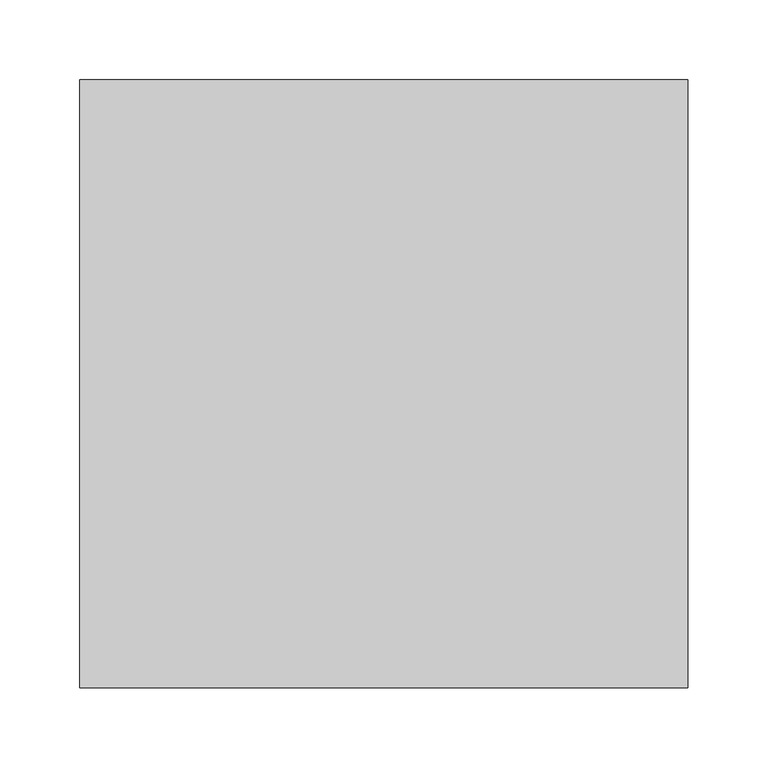
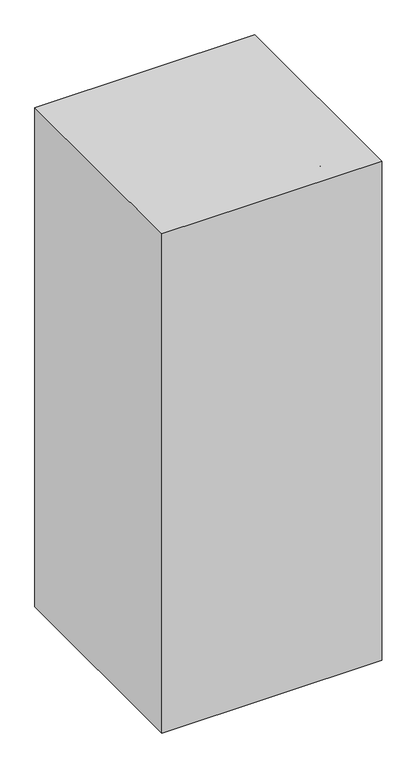
"""IFC4 building model written with IfcOpenShell, lengths in millimetres: proxy geometry, P2000 - Eyewash, Wall Mounted, Hands-Free : P2000 - Eyewash, Wall Mounted, Hands-Free."""

import ifcopenshell
import ifcopenshell.guid

model = None  # the IFC model being written
_history = None  # IfcOwnerHistory: only IFC2X3 demands one
_inside = {}  # id of a spatial element -> (the spatial element, [elements in it])
_under = {}  # id of a project, library or spatial element -> (it, [spatial elements below it])
_declared = {}  # id of a project -> (the project, [libraries it declares])
_typed = {}  # id of a type object -> (the type object, [elements of that type])
_made_of = {}  # id of a material, layer set ... -> (it, [elements and type objects made of it])


def new_model(schema):
    """Start an empty IFC model of exactly this schema.

    Asked for "IFC4X3", IfcOpenShell would pick the latest addendum, in which some entities
    have other attributes; the version numbers below select the first issue.
    IFC2X3 requires an IfcOwnerHistory on every rooted entity: one is made here for all.
    """
    global model, _history
    if schema == "IFC4X3":
        model = ifcopenshell.file(schema_version=(4, 3, 0, 0))
    else:
        model = ifcopenshell.file(schema=schema)
    _inside.clear()
    _under.clear()
    _declared.clear()
    _typed.clear()
    _made_of.clear()
    _history = None
    if model.schema == "IFC2X3":
        org = make("IfcOrganization", Name="unknown")
        user = make(
            "IfcPersonAndOrganization",
            ThePerson=make("IfcPerson", FamilyName="unknown"),
            TheOrganization=org,
        )
        app = make(
            "IfcApplication",
            ApplicationDeveloper=org,
            Version="unknown",
            ApplicationFullName="unknown",
            ApplicationIdentifier="unknown",
        )
        _history = make(
            "IfcOwnerHistory",
            OwningUser=user,
            OwningApplication=app,
            ChangeAction="ADDED",
            CreationDate=0,
        )
    return model


def make(cls, **values):
    """One entity of the class cls with the attributes given. An attribute that is None is left unset."""
    return model.create_entity(
        cls, **{name: value for name, value in values.items() if value is not None}
    )


def rooted(cls, **values):
    """An entity with a GlobalId (a new one), such as an element, a storey or a relation."""
    return make(cls, GlobalId=ifcopenshell.guid.new(), OwnerHistory=_history, **values)


def si_unit(unit_type, name, prefix=None):
    """IfcSIUnit, for example si_unit("LENGTHUNIT", "METRE", prefix="MILLI")."""
    return make("IfcSIUnit", UnitType=unit_type, Prefix=prefix, Name=name)


def assignment(units):
    """IfcUnitAssignment: the units of a project."""
    return None if units is None else make("IfcUnitAssignment", Units=units)


def point(xyz):
    """IfcCartesianPoint."""
    return None if xyz is None else make("IfcCartesianPoint", Coordinates=xyz)


def direction(xyz):
    """IfcDirection."""
    return None if xyz is None else make("IfcDirection", DirectionRatios=xyz)


def frame(location, z_axis=None, x_axis=None):
    """IfcAxis2Placement3D, a coordinate frame: its origin and axes. An axis left out is left unset."""
    return make(
        "IfcAxis2Placement3D",
        Location=point(location),
        Axis=direction(z_axis),
        RefDirection=direction(x_axis),
    )


def frame_2d(location, x_axis=None):
    """IfcAxis2Placement2D, a coordinate frame in the plane: its origin and x axis."""
    return make(
        "IfcAxis2Placement2D", Location=point(location), RefDirection=direction(x_axis)
    )


def origin():
    """The frame at (0, 0, 0) with its axes left unset."""
    return frame((0.0, 0.0, 0.0))


def origin_with_axes():
    """The frame at (0, 0, 0) with the z axis (0, 0, 1) and the x axis (1, 0, 0) written out."""
    return frame((0.0, 0.0, 0.0), z_axis=(0.0, 0.0, 1.0), x_axis=(1.0, 0.0, 0.0))


def place(relative_to, where):
    """IfcLocalPlacement: puts the frame where relative to a parent placement (None: the world)."""
    return make(
        "IfcLocalPlacement", PlacementRelTo=relative_to, RelativePlacement=where
    )


def context(
    kind, dimensions, precision=None, world=None, true_north=None, identifier=None
):
    """IfcGeometricRepresentationContext, for example the 3D "Model" context."""
    return make(
        "IfcGeometricRepresentationContext",
        ContextIdentifier=identifier,
        ContextType=kind,
        CoordinateSpaceDimension=dimensions,
        Precision=precision,
        WorldCoordinateSystem=world,
        TrueNorth=true_north,
    )


def project(units=None, contexts=None):
    """IfcProject with its units and contexts."""
    return rooted(
        "IfcProject",
        Name="project",
        RepresentationContexts=contexts,
        UnitsInContext=assignment(units),
    )


def spatial(cls, under=None, at=None, **own):
    """A site, building, storey or space (cls), placed at a placement, below another one or the project."""
    s = rooted(cls, ObjectPlacement=at, **own)
    if under is not None:
        _under.setdefault(under.id(), (under, []))[1].append(s)
    return s


def polyline(points):
    """IfcPolyline through the points."""
    return make("IfcPolyline", Points=[point(p) for p in points])


def circle_curve(where, radius):
    """IfcCircle in the frame where."""
    return make("IfcCircle", Position=where, Radius=radius)


def ellipse_curve(where, semi_axis1, semi_axis2):
    """IfcEllipse in the frame where."""
    return make(
        "IfcEllipse", Position=where, SemiAxis1=semi_axis1, SemiAxis2=semi_axis2
    )


def trimmed(basis, trim1, trim2, sense, master):
    """IfcTrimmedCurve: the piece of a basis curve between two trims."""
    return make(
        "IfcTrimmedCurve",
        BasisCurve=basis,
        Trim1=trim1,
        Trim2=trim2,
        SenseAgreement=sense,
        MasterRepresentation=master,
    )


def segment(curve, same_sense, transition):
    """IfcCompositeCurveSegment."""
    return make(
        "IfcCompositeCurveSegment",
        Transition=transition,
        SameSense=same_sense,
        ParentCurve=curve,
    )


def composite_curve(segments, self_intersect=None):
    """IfcCompositeCurve: segments joined end to end."""
    return make("IfcCompositeCurve", Segments=segments, SelfIntersect=self_intersect)


def outline(outer, holes=None, kind="AREA"):
    """IfcArbitraryClosedProfileDef: a profile drawn as a closed curve; with holes, ...WithVoids."""
    if holes is None:
        return make("IfcArbitraryClosedProfileDef", ProfileType=kind, OuterCurve=outer)
    return make(
        "IfcArbitraryProfileDefWithVoids",
        ProfileType=kind,
        OuterCurve=outer,
        InnerCurves=holes,
    )


def extrude(swept, where, along, depth):
    """IfcExtrudedAreaSolid: the profile swept, set in the frame where, extruded along a direction by depth."""
    return make(
        "IfcExtrudedAreaSolid",
        SweptArea=swept,
        Position=where,
        ExtrudedDirection=direction(along),
        Depth=depth,
    )


def shape(context_of_items, identifier, shape_type, items):
    """IfcShapeRepresentation: the items that make up one representation, for example the "Body"."""
    return make(
        "IfcShapeRepresentation",
        ContextOfItems=context_of_items,
        RepresentationIdentifier=identifier,
        RepresentationType=shape_type,
        Items=items,
    )


def source(mapping_origin, context_of_items, identifier, shape_type, items):
    """IfcRepresentationMap: a shape defined once, which mapped items show again and again."""
    return make(
        "IfcRepresentationMap",
        MappingOrigin=mapping_origin,
        MappedRepresentation=shape(context_of_items, identifier, shape_type, items),
    )


def transform(
    local_origin,
    x_axis=None,
    y_axis=None,
    z_axis=None,
    scale=None,
    scale2=None,
    scale3=None,
    uniform=True,
):
    """IfcCartesianTransformationOperator3D, or its non-uniform kind. x_axis, y_axis, z_axis: its Axis1, 2, 3."""
    if uniform:
        return make(
            "IfcCartesianTransformationOperator3D",
            Axis1=direction(x_axis),
            Axis2=direction(y_axis),
            LocalOrigin=point(local_origin),
            Scale=scale,
            Axis3=direction(z_axis),
        )
    return make(
        "IfcCartesianTransformationOperator3DnonUniform",
        Axis1=direction(x_axis),
        Axis2=direction(y_axis),
        LocalOrigin=point(local_origin),
        Scale=scale,
        Axis3=direction(z_axis),
        Scale2=scale2,
        Scale3=scale3,
    )


def mapped(mapping_source, mapping_target):
    """IfcMappedItem: shows the shape of a source again, moved by a transform."""
    return make(
        "IfcMappedItem", MappingSource=mapping_source, MappingTarget=mapping_target
    )


def made_of(thing, what):
    """Note that an element or type object is made of a material, layer set ...; save() writes the relation."""
    if what is not None:
        _made_of.setdefault(what.id(), (what, []))[1].append(thing)
    return thing


def element(
    cls,
    number,
    at=None,
    inside=None,
    cuts=None,
    type_object=None,
    material=None,
    context=None,
    identifier="Body",
    shape_type=None,
    held_by="IfcProductDefinitionShape",
    body=None,
    shapes=None,
    **own,
):
    """One element of the class cls, such as IfcWall. Its Tag is "e" and its number.

    at: its placement. inside: the storey or other place that contains it. cuts: it is an
    opening in that element (IfcRelVoidsElement). A single representation is given by context,
    identifier, shape_type and body (its items); several are given by shapes. held_by: the class
    of the entity that holds the representations. save() writes the other relations.
    """
    e = rooted(cls, Tag="e%d" % number, ObjectPlacement=at, **own)
    if body is not None:
        shapes = [shape(context, identifier, shape_type, body)]
    if shapes is not None:
        e.Representation = make(held_by, Representations=shapes)
    if inside is not None:
        _inside.setdefault(inside.id(), (inside, []))[1].append(e)
    if cuts is not None:
        rooted(
            "IfcRelVoidsElement", RelatingBuildingElement=cuts, RelatedOpeningElement=e
        )
    if type_object is not None:
        _typed.setdefault(type_object.id(), (type_object, []))[1].append(e)
    return made_of(e, material)


def aggregate(whole, parts):
    """IfcRelAggregates: a whole, such as a stair, and the parts it consists of."""
    return rooted("IfcRelAggregates", RelatingObject=whole, RelatedObjects=parts)


def save(model, path):
    """Write the relations noted so far, then the file.

    IfcRelAggregates (storeys below a building ...), IfcRelContainedInSpatialStructure (elements
    in a storey), IfcRelDefinesByType, IfcRelAssociatesMaterial and IfcRelDeclares: one each for
    every whole, place, type object, material and project.
    """
    for whole, parts in _under.values():
        aggregate(whole, parts)
    for where, things in _inside.values():
        rooted(
            "IfcRelContainedInSpatialStructure",
            RelatedElements=things,
            RelatingStructure=where,
        )
    for kind, things in _typed.values():
        rooted("IfcRelDefinesByType", RelatedObjects=things, RelatingType=kind)
    for what, things in _made_of.values():
        rooted("IfcRelAssociatesMaterial", RelatedObjects=things, RelatingMaterial=what)
    for by, libraries in _declared.values():
        rooted("IfcRelDeclares", RelatingContext=by, RelatedDefinitions=libraries)
    model.write(path)


def plane_surface(at):
    """IfcPlane: the flat surface through the origin of the frame at, square to its z axis."""
    return make("IfcPlane", Position=at)


def cylinder_surface(at, radius):
    """IfcCylindricalSurface: all points at the distance radius from the z axis of the frame at."""
    return make("IfcCylindricalSurface", Position=at, Radius=radius)


def revolved_surface(curve, axis_point, axis_direction):
    """IfcSurfaceOfRevolution: the curve turned about the line through axis_point along axis_direction."""
    return make(
        "IfcSurfaceOfRevolution",
        SweptCurve=make("IfcArbitraryOpenProfileDef", ProfileType="CURVE", Curve=curve),
        AxisPosition=make("IfcAxis1Placement", Location=point(axis_point), Axis=direction(axis_direction)),
    )


def advanced_brep(points, edges, surfaces, faces):
    """IfcAdvancedBrep: a solid bounded by faces that lie on surfaces and meet in shared edges.

    An edge is (start, end): straight between two places in points (the first is 0);
    or (start, end, curve); or (start, end, curve, False) where it runs against its curve.
    A face is (place in surfaces, loops), or (place, loops, False) where it looks against
    its surface's normal. A loop lists edges by number (the first is 1), with a minus sign
    where the edge is run from its end to its start. The first loop is the outer one.
    """
    corners = [point(p) for p in points]
    vertices = [make("IfcVertexPoint", VertexGeometry=c) for c in corners]
    made = []
    for start, end, *more in edges:
        made.append(
            make(
                "IfcEdgeCurve",
                EdgeStart=vertices[start],
                EdgeEnd=vertices[end],
                EdgeGeometry=more[0] if more else make("IfcPolyline", Points=[corners[start], corners[end]]),
                SameSense=more[1] if len(more) > 1 else True,
            )
        )
    hull = []
    for where, loops, *sense in faces:
        bounds = []
        for j, loop in enumerate(loops):
            ring = [make("IfcOrientedEdge", EdgeElement=made[abs(k) - 1], Orientation=k > 0) for k in loop]
            bounds.append(
                make(
                    "IfcFaceOuterBound" if j == 0 else "IfcFaceBound",
                    Bound=make("IfcEdgeLoop", EdgeList=ring),
                    Orientation=True,
                )
            )
        hull.append(make("IfcAdvancedFace", Bounds=bounds, FaceSurface=surfaces[where], SameSense=sense[0] if sense else True))
    return make("IfcAdvancedBrep", Outer=make("IfcClosedShell", CfsFaces=hull))


def specialty_equipment_1a8e0fdb(model_context):
    return source(origin(), model_context, "Body", "SolidModel", [
        extrude(outline(polyline([(0.0, -76.2), (0.0, 0.0), (12.7, 0.0), (12.7, -76.2), (0.0, -76.2)])), frame((-177.5900934, 239.9893842, 820.2504278), z_axis=(0.0, -0.4694715627858957, 0.8829475928589243), x_axis=(0.0, 0.8829475928589243, 0.4694715627858957)), (0.0, 0.0, 1.0), 76.2),
        advanced_brep(
        [(44.45, 215.9, 736.6), (44.45, 215.9, 723.9), (-16.0889464, 215.9, 736.6), (-22.0110536, 215.9, 723.9), (-78.0072211, 215.9, 810.3913264), (-90.7072211, 215.9, 805.7689044), (-78.0072211, 215.9, 858.8801154), (-90.7072211, 215.9, 846.1801154), (-160.5572211, 215.9, 858.8801154), (-160.5572211, 215.9, 846.1801154)],
        [
            (0, 1, circle_curve(frame((44.45, 215.9, 730.25), z_axis=(1.0, 0.0, 0.0), x_axis=(0.0, 0.0, -1.0)), 6.35)),
            (1, 0, circle_curve(frame((44.45, 215.9, 730.25), z_axis=(1.0, 0.0, 0.0), x_axis=(0.0, 0.0, -1.0)), 6.35)),
            (0, 2),
            (2, 3, ellipse_curve(frame((-19.05, 215.9, 730.25), z_axis=(0.9063077870366524, 0.0, -0.4226182617406946), x_axis=(0.42261826174069395, 0.0, 0.9063077870366525)), 7.0064498, 6.35)),
            (3, 1),
            (3, 2, ellipse_curve(frame((-19.05, 215.9, 730.25), z_axis=(0.9063077870366524, 0.0, -0.4226182617406946), x_axis=(0.42261826174069395, 0.0, 0.9063077870366525)), 7.0064498, 6.35)),
            (2, 4),
            (4, 5, ellipse_curve(frame((-84.3572211, 215.9, 808.0801154), z_axis=(0.3420201433256669, 0.0, -0.9396926207859092), x_axis=(0.9396926207859089, 0.0, 0.3420201433256674)), 6.7575289, 6.35)),
            (5, 3),
            (5, 4, ellipse_curve(frame((-84.3572211, 215.9, 808.0801154), z_axis=(0.3420201433256669, 0.0, -0.9396926207859092), x_axis=(0.9396926207859089, 0.0, 0.3420201433256674)), 6.7575289, 6.35)),
            (4, 6),
            (6, 7, ellipse_curve(frame((-84.3572211, 215.9, 852.5301154), z_axis=(0.7071067811865464, 0.0, -0.7071067811865487), x_axis=(-0.7071067811865487, 0.0, -0.7071067811865464)), 8.9802561, 6.35)),
            (7, 5),
            (7, 6, ellipse_curve(frame((-84.3572211, 215.9, 852.5301154), z_axis=(0.7071067811865464, 0.0, -0.7071067811865487), x_axis=(-0.7071067811865487, 0.0, -0.7071067811865464)), 8.9802561, 6.35)),
            (8, 9, circle_curve(frame((-160.5572211, 215.9, 852.5301154), z_axis=(-1.0, 0.0, 0.0), x_axis=(0.0, 0.0, -1.0)), 6.35)),
            (9, 8, circle_curve(frame((-160.5572211, 215.9, 852.5301154), z_axis=(-1.0, 0.0, 0.0), x_axis=(0.0, 0.0, -1.0)), 6.35)),
            (6, 8),
            (9, 7),
        ],
        [
            plane_surface(frame((44.45, 215.9, 730.25), z_axis=(1.0, 0.0, 0.0), x_axis=(0.0, -1.0, 0.0))),
            cylinder_surface(frame((44.45, 215.9, 730.25), z_axis=(1.0, 0.0, 0.0), x_axis=(0.0, 0.0, -1.0)), 6.35),
            cylinder_surface(frame((-19.05, 215.9, 730.25), z_axis=(0.6427876096865375, 0.0, -0.7660444431189797), x_axis=(-0.7660444431189797, 0.0, -0.6427876096865375)), 6.35),
            cylinder_surface(frame((-84.3572211, 215.9, 808.0801154), z_axis=(0.0, 0.0, -1.0), x_axis=(-1.0, 0.0, 0.0)), 6.35),
            plane_surface(frame((-160.5572211, 215.9, 852.5301154), z_axis=(-1.0, 0.0, 0.0), x_axis=(0.0, -1.0, 0.0))),
            cylinder_surface(frame((-84.3572211, 215.9, 852.5301154), z_axis=(1.0, 0.0, 0.0), x_axis=(0.0, 0.0, -1.0)), 6.35),
        ],
        [
            (0, [[1, 2]]),
            (1, [[-1, 3, 4, 5]]),
            (1, [[-2, -5, 6, -3]]),
            (2, [[-4, 7, 8, 9]]),
            (2, [[-6, -9, 10, -7]]),
            (3, [[-8, 11, 12, 13]]),
            (3, [[-10, -13, 14, -11]]),
            (4, [[15, 16]]),
            (5, [[-12, 17, -16, 18]]),
            (5, [[-14, -18, -15, -17]]),
        ],
    ),
        extrude(outline(composite_curve([segment(trimmed(circle_curve(frame_2d((730.25, 63.5)), 12.7), [point((730.25, 50.8))], [point((730.25, 76.2))], False, "CARTESIAN"), True, "CONTINUOUS"), segment(trimmed(circle_curve(frame_2d((730.25, 63.5)), 12.7), [point((730.25, 76.2))], [point((730.25, 50.8))], False, "CARTESIAN"), True, "CONTINUOUS")], self_intersect=False)), frame((0.0, 88.9, 0.0), z_axis=(0.0, 1.0, 0.0), x_axis=(0.0, 0.0, 1.0)), (0.0, 0.0, 1.0), 158.75),
        extrude(outline(composite_curve([segment(trimmed(circle_curve(frame_2d((730.25, 63.5)), 19.05), [point((730.25, 44.45))], [point((730.25, 82.55))], False, "CARTESIAN"), True, "CONTINUOUS"), segment(trimmed(circle_curve(frame_2d((730.25, 63.5)), 19.05), [point((730.25, 82.55))], [point((730.25, 44.45))], False, "CARTESIAN"), True, "CONTINUOUS")], self_intersect=False)), frame((0.0, 76.2, 0.0), z_axis=(0.0, 1.0, 0.0), x_axis=(0.0, 0.0, 1.0)), (0.0, 0.0, 1.0), 12.7),
        advanced_brep(
        [(6.6749119, 243.5968916, 875.3512512), (-10.6059042, 243.5968916, 883.409428), (-6.9449456, 243.5968916, 853.6764958), (-18.4550544, 243.5968916, 859.0437478)],
        [
            (0, 1, circle_curve(frame((-1.9654962, 243.5968916, 879.3803396), z_axis=(0.42261826174068884, 0.0, 0.9063077870366552), x_axis=(0.9063077870366554, 0.0, -0.4226182617406879)), 9.5336354)),
            (1, 0, circle_curve(frame((-1.9654962, 243.5968916, 879.3803396), z_axis=(0.42261826174068884, 0.0, 0.9063077870366552), x_axis=(-0.9063077870366548, 0.0, 0.42261826174068906)), 9.5336354)),
            (2, 3, circle_curve(frame((-12.7, 243.5968916, 856.3601218), z_axis=(-0.42261826174068884, 0.0, -0.9063077870366552), x_axis=(-0.9063077870366548, 0.0, 0.42261826174068906)), 6.35)),
            (3, 2, circle_curve(frame((-12.7, 243.5968916, 856.3601218), z_axis=(-0.42261826174068884, 0.0, -0.9063077870366552), x_axis=(0.9063077870366554, 0.0, -0.4226182617406879)), 6.35)),
            (2, 0),
            (1, 3),
        ],
        [
            plane_surface(frame((-1.9654962, 243.5968916, 879.3803396), z_axis=(0.42261826174068934, 0.0, 0.9063077870366547), x_axis=(0.0, 1.0, 0.0))),
            plane_surface(frame((-12.7, 243.5968916, 856.3601218), z_axis=(-0.42261826174068934, 0.0, -0.9063077870366547), x_axis=(0.0, 1.0, 0.0))),
            revolved_surface(polyline([(-6.9449455778731135, 243.5968916, 853.6764957896821), (6.674911899999998, 243.5968916, 875.3512512)]), (-34.1107742, 243.5968916, 810.4445683), (0.4226182617406887, 0.0, 0.9063077870366549)),
            revolved_surface(polyline([(-18.45505446296622, 243.5968916, 859.0437477089987), (-10.605904175746641, 243.5968916, 883.4094280752884)]), (-34.1107742, 243.5968916, 810.4445683), (0.4226182617406887, 0.0, 0.9063077870366549)),
        ],
        [
            (0, [[1, 2]]),
            (1, [[3, 4]]),
            (2, [[-3, 5, -2, 6]]),
            (3, [[-4, -6, -1, -5]]),
        ],
    ),
        advanced_brep(
        [(120.3250881, 243.5968916, 875.3512512), (137.6059042, 243.5968916, 883.409428), (133.9449456, 243.5968916, 853.6764958), (145.4550544, 243.5968916, 859.0437478)],
        [
            (0, 1, circle_curve(frame((128.9654962, 243.5968916, 879.3803396), z_axis=(-0.4226182617406885, 0.0, 0.9063077870366552), x_axis=(-0.9063077870366549, 0.0, -0.4226182617406886)), 9.5336354)),
            (1, 0, circle_curve(frame((128.9654962, 243.5968916, 879.3803396), z_axis=(-0.4226182617406885, 0.0, 0.9063077870366552), x_axis=(0.9063077870366556, 0.0, 0.42261826174068745)), 9.5336354)),
            (2, 3, circle_curve(frame((139.7, 243.5968916, 856.3601218), z_axis=(0.4226182617406885, 0.0, -0.9063077870366552), x_axis=(0.9063077870366556, 0.0, 0.42261826174068745)), 6.35)),
            (3, 2, circle_curve(frame((139.7, 243.5968916, 856.3601218), z_axis=(0.4226182617406885, 0.0, -0.9063077870366552), x_axis=(-0.9063077870366549, 0.0, -0.4226182617406886)), 6.35)),
            (3, 1),
            (0, 2),
        ],
        [
            plane_surface(frame((128.9654962, 243.5968916, 879.3803396), z_axis=(-0.42261826174068934, 0.0, 0.9063077870366547), x_axis=(0.0, -1.0, 0.0))),
            plane_surface(frame((139.7, 243.5968916, 856.3601218), z_axis=(0.42261826174068934, 0.0, -0.9063077870366547), x_axis=(0.0, -1.0, 0.0))),
            revolved_surface(polyline([(145.45505446296622, 243.5968916, 859.0437477089987), (137.60590417574664, 243.5968916, 883.4094280752884)]), (161.1107742, 243.5968916, 810.4445683), (-0.4226182617406885, 0.0, 0.9063077870366552)),
            revolved_surface(polyline([(133.9449455778731, 243.5968916, 853.676495789682), (120.3250881, 243.5968916, 875.3512512)]), (161.1107742, 243.5968916, 810.4445683), (-0.4226182617406885, 0.0, 0.9063077870366552)),
        ],
        [
            (0, [[1, 2]]),
            (1, [[3, 4]]),
            (2, [[-4, 5, -1, 6]]),
            (3, [[-3, -6, -2, -5]]),
        ],
    ),
        advanced_brep(
        [(133.9449456, 258.1987298, 853.6764958), (145.4550544, 258.1987298, 859.0437478), (140.7444281, 258.1987298, 839.0949585), (154.7573277, 258.1987298, 839.0949585), (127.603726, 258.1987298, 810.9146318), (135.6945183, 258.1987298, 798.2146318), (63.5, 258.1987298, 810.9146318), (63.5, 258.1987298, 798.2146318), (-0.603726, 258.1987298, 810.9146318), (-8.6945183, 258.1987298, 798.2146318), (-13.7444281, 258.1987298, 839.0949585), (-27.7573277, 258.1987298, 839.0949585), (-6.9449456, 258.1987298, 853.6764958), (-18.4550544, 258.1987298, 859.0437478)],
        [
            (0, 1, circle_curve(frame((139.7, 258.1987298, 856.3601218), z_axis=(-0.42261826174069717, 0.0, 0.906307787036651), x_axis=(0.906307787036651, 0.0, 0.42261826174069717)), 6.35)),
            (1, 0, circle_curve(frame((139.7, 258.1987298, 856.3601218), z_axis=(-0.42261826174069717, 0.0, 0.906307787036651), x_axis=(0.906307787036651, 0.0, 0.42261826174069717)), 6.35)),
            (0, 2),
            (2, 3, ellipse_curve(frame((147.7508779, 258.1987298, 839.0949585), z_axis=(0.0, 0.0, 1.0), x_axis=(-1.0, 0.0, 0.0)), 7.0064498, 6.35)),
            (3, 1),
            (3, 2, ellipse_curve(frame((147.7508779, 258.1987298, 839.0949585), z_axis=(0.0, 0.0, 1.0), x_axis=(-1.0, 0.0, 0.0)), 7.0064498, 6.35)),
            (2, 4),
            (4, 5, ellipse_curve(frame((131.6491221, 258.1987298, 804.5646318), z_axis=(0.8433914458128876, 0.0, 0.5372996083468209), x_axis=(-0.5372996083468209, 0.0, 0.8433914458128876)), 7.5291255, 6.35)),
            (5, 3),
            (5, 4, ellipse_curve(frame((131.6491221, 258.1987298, 804.5646318), z_axis=(0.8433914458128876, 0.0, 0.5372996083468209), x_axis=(-0.5372996083468209, 0.0, 0.8433914458128876)), 7.5291255, 6.35)),
            (4, 6),
            (6, 7, circle_curve(frame((63.5, 258.1987298, 804.5646318), z_axis=(1.0, 0.0, 0.0), x_axis=(0.0, 0.0, -1.0)), 6.35)),
            (7, 5),
            (7, 6, circle_curve(frame((63.5, 258.1987298, 804.5646318), z_axis=(1.0, 0.0, 0.0), x_axis=(0.0, 0.0, -1.0)), 6.35)),
            (6, 8),
            (8, 9, ellipse_curve(frame((-4.6491221, 258.1987298, 804.5646318), z_axis=(0.8433914458128859, 0.0, -0.5372996083468236), x_axis=(0.5372996083468233, 0.0, 0.8433914458128859)), 7.5291255, 6.35)),
            (9, 7),
            (9, 8, ellipse_curve(frame((-4.6491221, 258.1987298, 804.5646318), z_axis=(0.8433914458128859, 0.0, -0.5372996083468236), x_axis=(0.5372996083468233, 0.0, 0.8433914458128859)), 7.5291255, 6.35)),
            (8, 10),
            (10, 11, ellipse_curve(frame((-20.7508779, 258.1987298, 839.0949585), z_axis=(0.0, 0.0, -1.0), x_axis=(1.0, 0.0, 0.0)), 7.0064498, 6.35)),
            (11, 9),
            (11, 10, ellipse_curve(frame((-20.7508779, 258.1987298, 839.0949585), z_axis=(0.0, 0.0, -1.0), x_axis=(1.0, 0.0, 0.0)), 7.0064498, 6.35)),
            (12, 13, circle_curve(frame((-12.7, 258.1987298, 856.3601218), z_axis=(0.42261826174069733, 0.0, 0.9063077870366509), x_axis=(-0.9063077870366509, 0.0, 0.42261826174069733)), 6.35)),
            (13, 12, circle_curve(frame((-12.7, 258.1987298, 856.3601218), z_axis=(0.42261826174069733, 0.0, 0.9063077870366509), x_axis=(-0.9063077870366509, 0.0, 0.42261826174069733)), 6.35)),
            (10, 12),
            (13, 11),
        ],
        [
            plane_surface(frame((139.7, 76.2, 856.3601218), z_axis=(-0.42261826174069717, 0.0, 0.906307787036651), x_axis=(0.0, -1.0, 0.0))),
            cylinder_surface(frame((139.7, 258.1987298, 856.3601218), z_axis=(-0.42261826174069717, 0.0, 0.906307787036651), x_axis=(0.906307787036651, 0.0, 0.42261826174069717)), 6.35),
            cylinder_surface(frame((147.7508779, 258.1987298, 839.0949585), z_axis=(0.42261826174070577, 0.0, 0.9063077870366469), x_axis=(0.9063077870366469, 0.0, -0.42261826174070577)), 6.35),
            cylinder_surface(frame((131.6491221, 258.1987298, 804.5646318), z_axis=(1.0, 0.0, 0.0), x_axis=(0.0, 0.0, -1.0)), 6.35),
            cylinder_surface(frame((63.5, 258.1987298, 804.5646318), z_axis=(1.0, 0.0, 0.0), x_axis=(0.0, 0.0, -1.0)), 6.35),
            cylinder_surface(frame((-4.6491221, 258.1987298, 804.5646318), z_axis=(0.42261826174070016, 0.0, -0.9063077870366497), x_axis=(-0.9063077870366497, 0.0, -0.42261826174070016)), 6.35),
            plane_surface(frame((-12.7, 76.2, 856.3601218), z_axis=(0.4226182617406972, 0.0, 0.906307787036651), x_axis=(0.0, -1.0, 0.0))),
            cylinder_surface(frame((-20.7508779, 258.1987298, 839.0949585), z_axis=(-0.42261826174069733, 0.0, -0.9063077870366509), x_axis=(-0.9063077870366509, 0.0, 0.42261826174069733)), 6.35),
        ],
        [
            (0, [[1, 2]]),
            (1, [[-1, 3, 4, 5]]),
            (1, [[-2, -5, 6, -3]]),
            (2, [[-4, 7, 8, 9]]),
            (2, [[-6, -9, 10, -7]]),
            (3, [[-8, 11, 12, 13]]),
            (3, [[-10, -13, 14, -11]]),
            (4, [[-12, 15, 16, 17]]),
            (4, [[-14, -17, 18, -15]]),
            (5, [[-16, 19, 20, 21]]),
            (5, [[-18, -21, 22, -19]]),
            (6, [[23, 24]]),
            (7, [[-20, 25, -24, 26]]),
            (7, [[-22, -26, -23, -25]]),
        ],
    ),
        advanced_brep(
        [(-38.1, 254.0, 826.8645295), (165.1, 254.0, 826.8645295), (165.1, 254.0, 788.7645295), (-38.1, 254.0, 788.7645295), (-57.15, 254.0, 859.8600974), (184.15, 254.0, 859.8600974), (-52.5014774, 254.0, 864.50862), (179.5014774, 254.0, 864.50862), (-31.75, 254.0, 828.5660069), (158.75, 254.0, 828.5660069), (-31.75, 254.0, 795.1145295), (158.75, 254.0, 795.1145295), (63.5, 254.0, 795.1145295), (63.5, 254.0, 788.7645295)],
        [
            (0, 1, circle_curve(frame((63.5, 254.0, 826.8645295), z_axis=(0.0, 0.0, -1.0), x_axis=(1.0, 0.0, 0.0)), 101.6)),
            (1, 2),
            (2, 3, circle_curve(frame((63.5, 254.0, 788.7645295), z_axis=(0.0, 0.0, 1.0), x_axis=(1.0, 0.0, 0.0)), 101.6)),
            (3, 0),
            (1, 0, circle_curve(frame((63.5, 254.0, 826.8645295), z_axis=(0.0, 0.0, -1.0), x_axis=(1.0, 0.0, 0.0)), 101.6)),
            (3, 2, circle_curve(frame((63.5, 254.0, 788.7645295), z_axis=(0.0, 0.0, 1.0), x_axis=(1.0, 0.0, 0.0)), 101.6)),
            (4, 5, circle_curve(frame((63.5, 254.0, 859.8600974), z_axis=(0.0, 0.0, -1.0), x_axis=(1.0, 0.0, 0.0)), 120.65)),
            (5, 1),
            (0, 4),
            (5, 4, circle_curve(frame((63.5, 254.0, 859.8600974), z_axis=(0.0, 0.0, -1.0), x_axis=(1.0, 0.0, 0.0)), 120.65)),
            (6, 7, circle_curve(frame((63.5, 254.0, 864.50862), z_axis=(0.0, 0.0, -1.0), x_axis=(1.0, 0.0, 0.0)), 116.0014774)),
            (7, 5),
            (4, 6),
            (7, 6, circle_curve(frame((63.5, 254.0, 864.50862), z_axis=(0.0, 0.0, -1.0), x_axis=(1.0, 0.0, 0.0)), 116.0014774)),
            (8, 9, circle_curve(frame((63.5, 254.0, 828.5660069), z_axis=(0.0, 0.0, -1.0), x_axis=(1.0, 0.0, 0.0)), 95.25)),
            (9, 7),
            (6, 8),
            (9, 8, circle_curve(frame((63.5, 254.0, 828.5660069), z_axis=(0.0, 0.0, -1.0), x_axis=(1.0, 0.0, 0.0)), 95.25)),
            (10, 11, circle_curve(frame((63.5, 254.0, 795.1145295), z_axis=(0.0, 0.0, -1.0), x_axis=(1.0, 0.0, 0.0)), 95.25)),
            (11, 9),
            (8, 10),
            (11, 10, circle_curve(frame((63.5, 254.0, 795.1145295), z_axis=(0.0, 0.0, -1.0), x_axis=(1.0, 0.0, 0.0)), 95.25)),
            (12, 11),
            (10, 12),
            (2, 13),
            (13, 3),
        ],
        [
            cylinder_surface(frame((63.5, 254.0, 884.0145295), z_axis=(0.0, 0.0, 1.0), x_axis=(1.0, 0.0, 0.0)), 101.6),
            revolved_surface(polyline([(165.1, 254.0, 826.8645295), (184.15, 254.0, 859.8600974)]), (63.5, 254.0, 884.0145295), (0.0, 0.0, 1.0)),
            revolved_surface(polyline([(184.15, 254.0, 859.8600974), (179.5014774, 254.0, 864.50862)]), (63.5, 254.0, 884.0145295), (0.0, 0.0, 1.0)),
            revolved_surface(polyline([(179.5014774, 254.0, 864.50862), (158.75, 254.0, 828.5660069)]), (63.5, 254.0, 884.0145295), (0.0, 0.0, 1.0)),
            revolved_surface(polyline([(158.75, 254.0, 828.5660069), (158.75, 254.0, 795.1145295)]), (63.5, 254.0, 884.0145295), (0.0, 0.0, 1.0)),
            plane_surface(frame((63.5, 254.0, 795.1145295), z_axis=(0.0, 0.0, 1.0), x_axis=(1.0, 0.0, 0.0))),
            plane_surface(frame((63.5, 254.0, 788.7645295), z_axis=(0.0, 0.0, -1.0), x_axis=(1.0, 0.0, 0.0))),
        ],
        [
            (0, [[1, 2, 3, 4]]),
            (0, [[5, -4, 6, -2]]),
            (1, [[7, 8, -1, 9]]),
            (1, [[10, -9, -5, -8]]),
            (2, [[11, 12, -7, 13]]),
            (2, [[14, -13, -10, -12]]),
            (3, [[15, 16, -11, 17]]),
            (3, [[18, -17, -14, -16]]),
            (4, [[19, 20, -15, 21]]),
            (4, [[22, -21, -18, -20]]),
            (5, [[23, -19, 24]]),
            (5, [[-24, -22, -23]]),
            (6, [[-3, 25, 26]]),
            (6, [[-6, -26, -25]]),
        ],
    ),
        extrude(outline(composite_curve([segment(trimmed(circle_curve(frame_2d((63.5, 242.7630601)), 19.05), [point((44.45, 242.7630601))], [point((82.55, 242.7630601))], False, "CARTESIAN"), True, "CONTINUOUS"), segment(trimmed(circle_curve(frame_2d((63.5, 242.7630601)), 19.05), [point((82.55, 242.7630601))], [point((44.45, 242.7630601))], False, "CARTESIAN"), True, "CONTINUOUS")], self_intersect=False)), frame((0.0, 0.0, 678.0316343), z_axis=(0.0, 0.0, 1.0), x_axis=(1.0, 0.0, 0.0)), (0.0, 0.0, 1.0), 110.7328952),
        extrude(outline(polyline([(190.5, 442.9125), (190.5, 61.9125), (-190.5, 61.9125), (-190.5, 442.9125), (190.5, 442.9125)])), origin_with_axes(), (0.0, 0.0, 1.0), 914.4),
    ])


if __name__ == "__main__":
    model = new_model("IFC4")
    model_context = context("Model", 3, world=origin())
    ifc_project = project(units=[si_unit("LENGTHUNIT", "METRE", prefix="MILLI")], contexts=[model_context])
    site = spatial("IfcSite", under=ifc_project)
    building = spatial("IfcBuilding", under=site)
    placement = place(None, origin())
    specialty_equipment_shape = specialty_equipment_1a8e0fdb(model_context)
    element("IfcBuildingElementProxy", 1, Name="P2000 - Eyewash, Wall Mounted, Hands-Free : P2000 - Eyewash, Wall Mounted, Hands-Free", ObjectType="P2000 - Eyewash, Wall Mounted, Hands-Free : P2000 - Eyewash, Wall Mounted, Hands-Free", at=placement, inside=building, context=model_context, shape_type="MappedRepresentation", body=[
        mapped(specialty_equipment_shape, transform((0.0, 0.0, 0.0), x_axis=(1.0, 0.0, 0.0), y_axis=(0.0, 1.0, 0.0), z_axis=(0.0, 0.0, 1.0))),
    ])
    save(model, "model.ifc")

# Revit data of these elements
# Project information
#   Sheets - Total = "6"
#   Project Issue Date = "Issue Date"
#   Project Status = "Project Status"
#   Client Name = "Owner"
#   Project Address = "Enter address here"
#   Project Name = "Project Name"
#   Project Number = "Project Number"
#   Publication Date = "30-Jan-15"
# Type "P2000 - Eyewash, Wall Mounted, Hands-Free : P2000 - Eyewash, Wall Mounted, Hands-Free"
#   Watts2 = "0"
#   Watts1 = "0"
#   Unit_Issue = "EA"
#   UTIL_6_Misc = "-"
#   UTIL_5_NonMedGas = "-"
#   UTIL_4_MiscGas = "-"
#   UTIL_3_MedGas = "-"
#   UTIL_2_Elec = "-"
#   UTIL_1_WaterDrain = "B"
#   Nomenclature = "Eyewash, Wall Mounted, Hands-Free"
#   NSN = "4510"
#   Location [instance default] = ""
#   JSN = "P2000"
#   Fund_Source_VA = "-"
#   Fund_Source_Navy = "-"
#   Fund_Source_Army = "-"
#   Fund_Source_AF = "-"
#   ELEC_Volts2 = "0"
#   ELEC_Volts1 = "0"
#   ELEC_Phase2 = "0"
#   ELEC_Phase1 = "0"
#   ELEC_HertzSwitch = "0"
#   ELEC_HertzDependent = "0"
#   ELEC_Hertz = "0"
#   ELEC_Amps2 = "0"
#   ELEC_Amps1 = "0"
#   DetailDescription = "Wall mounted emergency eye wash station. The flow of water from the unit is activated by hand. Upon initiation of water flow the unit will operate hands free to provide streams of water to clear foreign particles or dilute caustic liquids from the eyes in emergency situations. Used in laboratories and areas of the hospital where employees are subject to foreign bodies or liquid material to the eyes."
#   CAT_VA = "A"
#   CAT_Navy = "A"
#   CAT_IHS = "-"
#   CAT_Army = "A"
#   CAT_AF = "A"
#   BTUperhour = "0"
#   Weight_IP = 8
#   DIM_Width_IP = 1' - 3"
#   DIM_Height_IP = 3' - 0"
#   DIM_Depth_IP = 1' - 3"
# Element 1 (IfcBuildingElementProxy, "P2000 - Eyewash, Wall Mounted, Hands-Free : P2000 - Eyewash, Wall Mounted, Hands-Free")
#   Location = "UCCL2"
#   Materials on its faces: "EquipSpace"
# Materials
#   "EquipSpace": class "Unassigned", colour RGB 221 217 195, transparency 0.5
